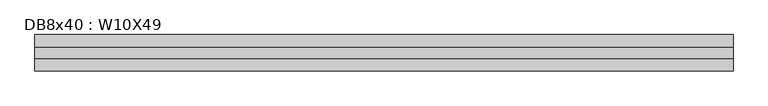
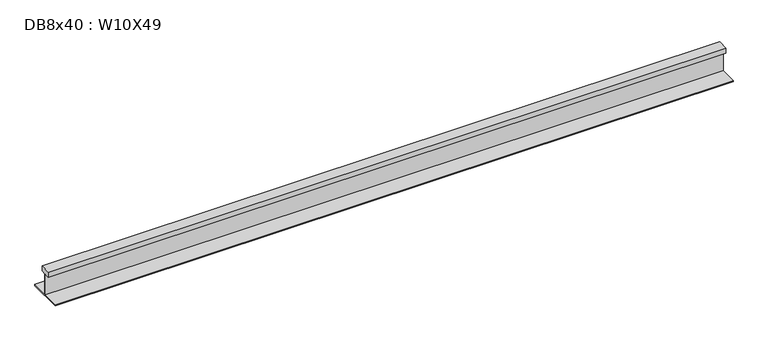
"""IFC4 building model written with IfcOpenShell, lengths in millimetres: beam geometry, DB8x40 : W10X49."""

from ifc_helpers import new_model, si_unit, frame, origin, place, context, project, spatial, polyline, outline, extrude, source, transform, mapped, element, save


def db8x40_w10x49_f7015ab1(model_context):
    return source(origin(), model_context, "Body", "SweptSolid", [
        extrude(outline(polyline([(38.1, 144.3355), (38.1, 106.2355), (2.921, 106.2355), (2.921, -49.53), (127.0, -49.53), (127.0, -59.182), (-127.0, -59.182), (-127.0, -49.53), (-2.921, -49.53), (-2.921, 106.2355), (-38.1, 106.2355), (-38.1, 144.3355), (38.1, 144.3355)])), frame((-2441.829, 0.0, 0.0), z_axis=(1.0, 0.0, 0.0), x_axis=(0.0, 1.0, 0.0)), (0.0, 0.0, 1.0), 4883.658),
    ])


if __name__ == "__main__":
    model = new_model("IFC4")
    model_context = context("Model", 3, world=origin())
    ifc_project = project(units=[si_unit("LENGTHUNIT", "METRE", prefix="MILLI")], contexts=[model_context])
    site = spatial("IfcSite", under=ifc_project)
    building = spatial("IfcBuilding", under=site)
    placement = place(None, origin())
    db8x40_w10x49_shape = db8x40_w10x49_f7015ab1(model_context)
    element("IfcBeam", 1, ObjectType="DB8x40 : W10X49", at=placement, inside=building, context=model_context, shape_type="MappedRepresentation", body=[
        mapped(db8x40_w10x49_shape, transform((0.0, 0.0, 0.0), x_axis=(1.0, 0.0, 0.0), y_axis=(0.0, 1.0, 0.0), z_axis=(0.0, 0.0, 1.0))),
    ])
    save(model, "model.ifc")

# Revit data of these elements
# Type "DB8x40 : W10X49"
#   Assembly Code = "B10"
#   W = 53
#   Length [instance default] = 5' - 0"
#   bf = 0' - 10"
#   d = 1' - 0.1"
#   k = 0' - 1 3/8"
#   k2 = 0' - 0.8"
#   tf = 0' - 0.575"
#   tw = 0' - 0.345"
#   A = 0.108333 SF
#   Structural Material [instance default] = Steel ASTM A992
# Element 1 (IfcBeam, "DB8x40 : W10X49")
#   Materials on its faces: "Steel ASTM A992"
# Materials
#   "Steel ASTM A992": class "Metal", colour RGB 199 199 199, transparency 0, Description = "Structural steel 50ksi", Cost = 0
